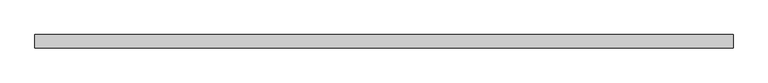
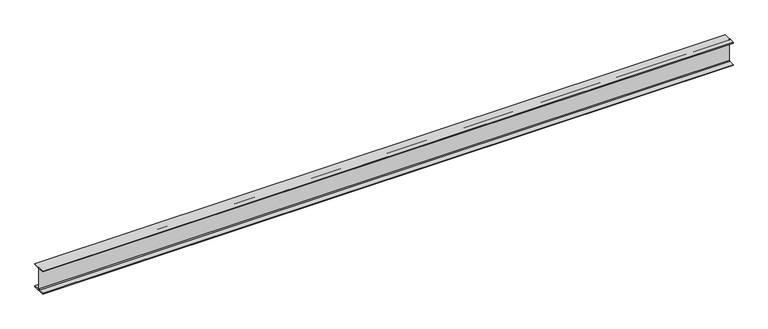
"""IFC4 building model written with IfcOpenShell, lengths in millimetres: beam geometry, Old_Steel Beam_H-KSD3502 : H_SB_ASB_H-300×300x10x15."""

from ifc_helpers import new_model, si_unit, point, frame, frame_2d, origin, place, context, project, spatial, polyline, circle_curve, trimmed, segment, composite_curve, outline, extrude, source, transform, mapped, element, save


def beam_44e4a88d(model_context):
    return source(origin(), model_context, "Body", "SweptSolid", [
        extrude(outline(composite_curve([segment(polyline([(82.5, -141.5), (82.5, -151.7), (-82.5, -151.7), (-82.5, -141.5), (-11.9, -141.5)]), True, "CONTINUOUS"), segment(trimmed(circle_curve(frame_2d((-11.9, -132.6)), 8.9), [point((-11.9, -141.5))], [point((-3.0, -132.6))], True, "CARTESIAN"), True, "CONTINUOUS"), segment(polyline([(-3.0, -132.6), (-3.0, 132.6)]), True, "CONTINUOUS"), segment(trimmed(circle_curve(frame_2d((-11.9, 132.6)), 8.9), [point((-3.0, 132.6))], [point((-11.9, 141.5))], True, "CARTESIAN"), True, "CONTINUOUS"), segment(polyline([(-11.9, 141.5), (-82.5, 141.5), (-82.5, 151.7), (82.5, 151.7), (82.5, 141.5), (11.9, 141.5)]), True, "CONTINUOUS"), segment(trimmed(circle_curve(frame_2d((11.9, 132.6)), 8.9), [point((11.9, 141.5))], [point((3.0, 132.6))], True, "CARTESIAN"), True, "CONTINUOUS"), segment(polyline([(3.0, 132.6), (3.0, -132.6)]), True, "CONTINUOUS"), segment(trimmed(circle_curve(frame_2d((11.9, -132.6)), 8.9), [point((3.0, -132.6))], [point((11.9, -141.5))], True, "CARTESIAN"), True, "CONTINUOUS"), segment(polyline([(11.9, -141.5), (82.5, -141.5)]), True, "CONTINUOUS")], self_intersect=False)), frame((-4374.2452733, 0.0, 0.0), z_axis=(1.0, 0.0, 0.0), x_axis=(0.0, 1.0, 0.0)), (0.0, 0.0, 1.0), 8647.1704515),
    ])


if __name__ == "__main__":
    model = new_model("IFC4")
    model_context = context("Model", 3, world=origin())
    ifc_project = project(units=[si_unit("LENGTHUNIT", "METRE", prefix="MILLI")], contexts=[model_context])
    site = spatial("IfcSite", under=ifc_project)
    building = spatial("IfcBuilding", under=site)
    placement = place(None, origin())
    beam_shape = beam_44e4a88d(model_context)
    element("IfcBeam", 1, ObjectType="Old_Steel Beam_H-KSD3502 : H_SB_ASB_H-300×300x10x15", at=placement, inside=building, context=model_context, shape_type="MappedRepresentation", body=[
        mapped(beam_shape, transform((0.0, 0.0, 0.0), x_axis=(1.0, 0.0, 0.0), y_axis=(0.0, 1.0, 0.0), z_axis=(0.0, 0.0, 1.0))),
    ])
    save(model, "model.ifc")

# Revit data of these elements
# Type "Old_Steel Beam_H-KSD3502 : H_SB_ASB_H-300×300x10x15"
#   Width = 30.0 cm
#   Web Thickness = 1.0 cm
#   Web Fillet = 1.8 cm
#   Warping Constant = 1370670.0 cm⁶
#   Torsional Moment of Inertia = 77.00 cm⁴
#   Torsional Modulus = 1.0 cm³
#   Section Area = 119.8 cm²
#   Plastic Modulus weak axis = 684.0 cm³
#   Plastic Modulus strong axis = 1500.0 cm³
#   Perimeter = 1.75 m²/m
#   Nominal Weight = 94.00 kgf/m
#   Moment of Inertia weak axis = 6750.00 cm⁴
#   Moment of Inertia strong axis = 20400.00 cm⁴
#   Height = 30.0 cm
#   Flange Thickness = 1.5 cm
#   Elastic Modulus weak axis = 450.0 cm³
#   Elastic Modulus strong axis = 1360.0 cm³
#   Centroid Vertical = 15.0 cm
#   Centroid Horizontal = 15.0 cm
#   Length [instance default] = 1.5240 m
#   Structural Material [instance default] = Steel, 45-345
#   Assembly Code = ""
# Element 1 (IfcBeam, "Old_Steel Beam_H-KSD3502 : H_SB_ASB_H-300×300x10x15")
#   Structural Material = none
# Materials
#   "Steel, 45-345": class "Metal", colour RGB 189 187 185, transparency 0, Description = "Steel 345 MPa", Cost = 0
